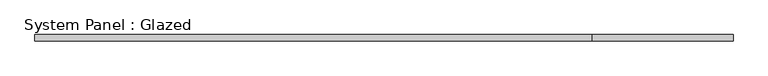
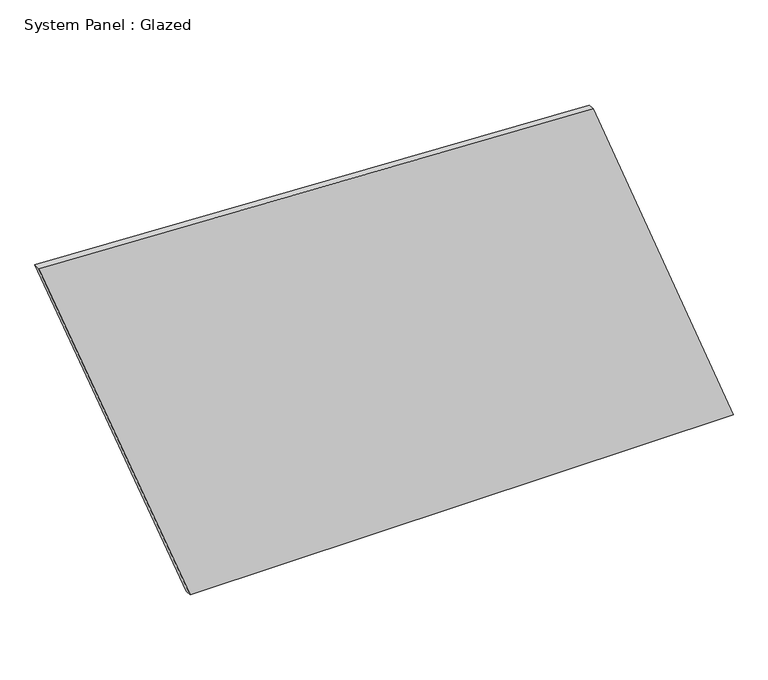
"""IFC4 building model written with IfcOpenShell, lengths in millimetres: plate geometry, System Panel : Glazed."""

from ifc_helpers import new_model, si_unit, frame, origin, place, context, project, spatial, polyline, outline, extrude, source, transform, mapped, element, save


def system_panel_glazed_ea40fa90(model_context):
    return source(origin(), model_context, "Body", "SweptSolid", [
        extrude(outline(polyline([(0.0, -761.7705902), (0.0, 1351.5772098), (1450.4840303, 806.3458623), (1548.8876781, -1351.5772098), (0.0, -761.7705902)])), frame((0.0, -49.5, 0.0), z_axis=(0.0, 1.0, 0.0), x_axis=(0.0, 0.0, 1.0)), (0.0, 0.0, 1.0), 25.0),
    ])


if __name__ == "__main__":
    model = new_model("IFC4")
    model_context = context("Model", 3, world=origin())
    ifc_project = project(units=[si_unit("LENGTHUNIT", "METRE", prefix="MILLI")], contexts=[model_context])
    site = spatial("IfcSite", under=ifc_project)
    building = spatial("IfcBuilding", under=site)
    placement = place(None, origin())
    system_panel_glazed_shape = system_panel_glazed_ea40fa90(model_context)
    element("IfcPlate", 1, ObjectType="System Panel : Glazed", at=placement, inside=building, context=model_context, shape_type="MappedRepresentation", body=[
        mapped(system_panel_glazed_shape, transform((0.0, 0.0, 0.0), x_axis=(1.0, 0.0, 0.0), y_axis=(0.0, 1.0, 0.0), z_axis=(0.0, 0.0, 1.0))),
    ])
    save(model, "model.ifc")

# Revit data of these elements
# Element 1 (IfcPlate, "System Panel : Glazed")
#   Materials on its faces: "Glass, Clear Glazing"
# Materials
#   "Glass, Clear Glazing": class "Glass", colour RGB 247 249 248, transparency 0.85, Description = "Clear glazing", Cost = 0
